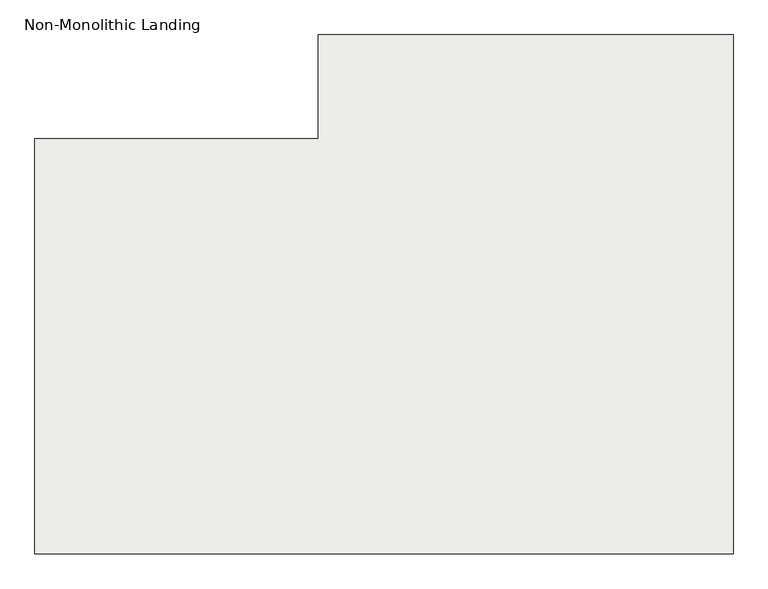
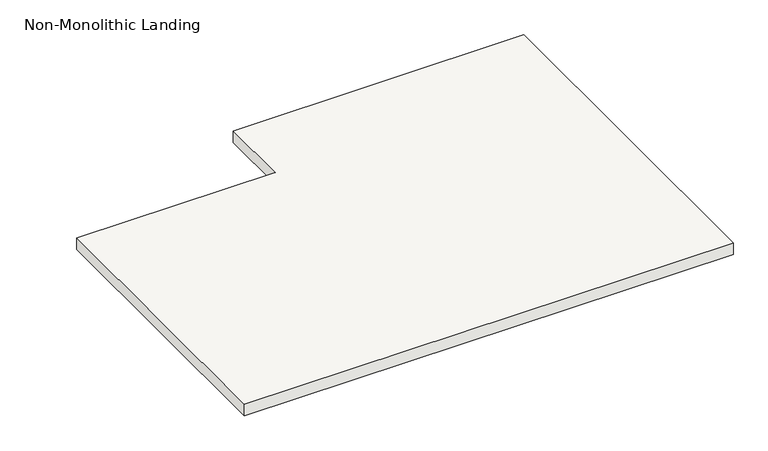
"""IFC4 building model written with IfcOpenShell, lengths in millimetres: slab geometry, Non-Monolithic Landing."""

import ifcopenshell
import ifcopenshell.guid

model = None  # the IFC model being written
_history = None  # IfcOwnerHistory: only IFC2X3 demands one
_inside = {}  # id of a spatial element -> (the spatial element, [elements in it])
_under = {}  # id of a project, library or spatial element -> (it, [spatial elements below it])
_declared = {}  # id of a project -> (the project, [libraries it declares])
_typed = {}  # id of a type object -> (the type object, [elements of that type])
_made_of = {}  # id of a material, layer set ... -> (it, [elements and type objects made of it])


def new_model(schema):
    """Start an empty IFC model of exactly this schema.

    Asked for "IFC4X3", IfcOpenShell would pick the latest addendum, in which some entities
    have other attributes; the version numbers below select the first issue.
    IFC2X3 requires an IfcOwnerHistory on every rooted entity: one is made here for all.
    """
    global model, _history
    if schema == "IFC4X3":
        model = ifcopenshell.file(schema_version=(4, 3, 0, 0))
    else:
        model = ifcopenshell.file(schema=schema)
    _inside.clear()
    _under.clear()
    _declared.clear()
    _typed.clear()
    _made_of.clear()
    _history = None
    if model.schema == "IFC2X3":
        org = make("IfcOrganization", Name="unknown")
        user = make(
            "IfcPersonAndOrganization",
            ThePerson=make("IfcPerson", FamilyName="unknown"),
            TheOrganization=org,
        )
        app = make(
            "IfcApplication",
            ApplicationDeveloper=org,
            Version="unknown",
            ApplicationFullName="unknown",
            ApplicationIdentifier="unknown",
        )
        _history = make(
            "IfcOwnerHistory",
            OwningUser=user,
            OwningApplication=app,
            ChangeAction="ADDED",
            CreationDate=0,
        )
    return model


def make(cls, **values):
    """One entity of the class cls with the attributes given. An attribute that is None is left unset."""
    return model.create_entity(
        cls, **{name: value for name, value in values.items() if value is not None}
    )


def rooted(cls, **values):
    """An entity with a GlobalId (a new one), such as an element, a storey or a relation."""
    return make(cls, GlobalId=ifcopenshell.guid.new(), OwnerHistory=_history, **values)


def si_unit(unit_type, name, prefix=None):
    """IfcSIUnit, for example si_unit("LENGTHUNIT", "METRE", prefix="MILLI")."""
    return make("IfcSIUnit", UnitType=unit_type, Prefix=prefix, Name=name)


def assignment(units):
    """IfcUnitAssignment: the units of a project."""
    return None if units is None else make("IfcUnitAssignment", Units=units)


def point(xyz):
    """IfcCartesianPoint."""
    return None if xyz is None else make("IfcCartesianPoint", Coordinates=xyz)


def direction(xyz):
    """IfcDirection."""
    return None if xyz is None else make("IfcDirection", DirectionRatios=xyz)


def frame(location, z_axis=None, x_axis=None):
    """IfcAxis2Placement3D, a coordinate frame: its origin and axes. An axis left out is left unset."""
    return make(
        "IfcAxis2Placement3D",
        Location=point(location),
        Axis=direction(z_axis),
        RefDirection=direction(x_axis),
    )


def origin():
    """The frame at (0, 0, 0) with its axes left unset."""
    return frame((0.0, 0.0, 0.0))


def place(relative_to, where):
    """IfcLocalPlacement: puts the frame where relative to a parent placement (None: the world)."""
    return make(
        "IfcLocalPlacement", PlacementRelTo=relative_to, RelativePlacement=where
    )


def context(
    kind, dimensions, precision=None, world=None, true_north=None, identifier=None
):
    """IfcGeometricRepresentationContext, for example the 3D "Model" context."""
    return make(
        "IfcGeometricRepresentationContext",
        ContextIdentifier=identifier,
        ContextType=kind,
        CoordinateSpaceDimension=dimensions,
        Precision=precision,
        WorldCoordinateSystem=world,
        TrueNorth=true_north,
    )


def project(units=None, contexts=None):
    """IfcProject with its units and contexts."""
    return rooted(
        "IfcProject",
        Name="project",
        RepresentationContexts=contexts,
        UnitsInContext=assignment(units),
    )


def spatial(cls, under=None, at=None, **own):
    """A site, building, storey or space (cls), placed at a placement, below another one or the project."""
    s = rooted(cls, ObjectPlacement=at, **own)
    if under is not None:
        _under.setdefault(under.id(), (under, []))[1].append(s)
    return s


def polyline(points):
    """IfcPolyline through the points."""
    return make("IfcPolyline", Points=[point(p) for p in points])


def outline(outer, holes=None, kind="AREA"):
    """IfcArbitraryClosedProfileDef: a profile drawn as a closed curve; with holes, ...WithVoids."""
    if holes is None:
        return make("IfcArbitraryClosedProfileDef", ProfileType=kind, OuterCurve=outer)
    return make(
        "IfcArbitraryProfileDefWithVoids",
        ProfileType=kind,
        OuterCurve=outer,
        InnerCurves=holes,
    )


def extrude(swept, where, along, depth):
    """IfcExtrudedAreaSolid: the profile swept, set in the frame where, extruded along a direction by depth."""
    return make(
        "IfcExtrudedAreaSolid",
        SweptArea=swept,
        Position=where,
        ExtrudedDirection=direction(along),
        Depth=depth,
    )


def shape(context_of_items, identifier, shape_type, items):
    """IfcShapeRepresentation: the items that make up one representation, for example the "Body"."""
    return make(
        "IfcShapeRepresentation",
        ContextOfItems=context_of_items,
        RepresentationIdentifier=identifier,
        RepresentationType=shape_type,
        Items=items,
    )


def source(mapping_origin, context_of_items, identifier, shape_type, items):
    """IfcRepresentationMap: a shape defined once, which mapped items show again and again."""
    return make(
        "IfcRepresentationMap",
        MappingOrigin=mapping_origin,
        MappedRepresentation=shape(context_of_items, identifier, shape_type, items),
    )


def transform(
    local_origin,
    x_axis=None,
    y_axis=None,
    z_axis=None,
    scale=None,
    scale2=None,
    scale3=None,
    uniform=True,
):
    """IfcCartesianTransformationOperator3D, or its non-uniform kind. x_axis, y_axis, z_axis: its Axis1, 2, 3."""
    if uniform:
        return make(
            "IfcCartesianTransformationOperator3D",
            Axis1=direction(x_axis),
            Axis2=direction(y_axis),
            LocalOrigin=point(local_origin),
            Scale=scale,
            Axis3=direction(z_axis),
        )
    return make(
        "IfcCartesianTransformationOperator3DnonUniform",
        Axis1=direction(x_axis),
        Axis2=direction(y_axis),
        LocalOrigin=point(local_origin),
        Scale=scale,
        Axis3=direction(z_axis),
        Scale2=scale2,
        Scale3=scale3,
    )


def mapped(mapping_source, mapping_target):
    """IfcMappedItem: shows the shape of a source again, moved by a transform."""
    return make(
        "IfcMappedItem", MappingSource=mapping_source, MappingTarget=mapping_target
    )


def made_of(thing, what):
    """Note that an element or type object is made of a material, layer set ...; save() writes the relation."""
    if what is not None:
        _made_of.setdefault(what.id(), (what, []))[1].append(thing)
    return thing


def element(
    cls,
    number,
    at=None,
    inside=None,
    cuts=None,
    type_object=None,
    material=None,
    context=None,
    identifier="Body",
    shape_type=None,
    held_by="IfcProductDefinitionShape",
    body=None,
    shapes=None,
    **own,
):
    """One element of the class cls, such as IfcWall. Its Tag is "e" and its number.

    at: its placement. inside: the storey or other place that contains it. cuts: it is an
    opening in that element (IfcRelVoidsElement). A single representation is given by context,
    identifier, shape_type and body (its items); several are given by shapes. held_by: the class
    of the entity that holds the representations. save() writes the other relations.
    """
    e = rooted(cls, Tag="e%d" % number, ObjectPlacement=at, **own)
    if body is not None:
        shapes = [shape(context, identifier, shape_type, body)]
    if shapes is not None:
        e.Representation = make(held_by, Representations=shapes)
    if inside is not None:
        _inside.setdefault(inside.id(), (inside, []))[1].append(e)
    if cuts is not None:
        rooted(
            "IfcRelVoidsElement", RelatingBuildingElement=cuts, RelatedOpeningElement=e
        )
    if type_object is not None:
        _typed.setdefault(type_object.id(), (type_object, []))[1].append(e)
    return made_of(e, material)


def aggregate(whole, parts):
    """IfcRelAggregates: a whole, such as a stair, and the parts it consists of."""
    return rooted("IfcRelAggregates", RelatingObject=whole, RelatedObjects=parts)


def save(model, path):
    """Write the relations noted so far, then the file.

    IfcRelAggregates (storeys below a building ...), IfcRelContainedInSpatialStructure (elements
    in a storey), IfcRelDefinesByType, IfcRelAssociatesMaterial and IfcRelDeclares: one each for
    every whole, place, type object, material and project.
    """
    for whole, parts in _under.values():
        aggregate(whole, parts)
    for where, things in _inside.values():
        rooted(
            "IfcRelContainedInSpatialStructure",
            RelatedElements=things,
            RelatingStructure=where,
        )
    for kind, things in _typed.values():
        rooted("IfcRelDefinesByType", RelatedObjects=things, RelatingType=kind)
    for what, things in _made_of.values():
        rooted("IfcRelAssociatesMaterial", RelatedObjects=things, RelatingMaterial=what)
    for by, libraries in _declared.values():
        rooted("IfcRelDeclares", RelatingContext=by, RelatedDefinitions=libraries)
    model.write(path)


def non_monolithic_landing_fffc1bba(model_context):
    return source(origin(), model_context, "Body", "SweptSolid", [
        extrude(outline(polyline([(22758.5156953, -2193.8863261), (22758.5156953, -3693.8863261), (20739.4907974, -3693.8863261), (20739.4907974, -2493.8863261), (21558.5156953, -2493.8863261), (21558.5156953, -2193.8863261), (22758.5156953, -2193.8863261)])), frame((0.0, 0.0, 1450.0), z_axis=(0.0, 0.0, 1.0), x_axis=(1.0, 0.0, 0.0)), (0.0, 0.0, 1.0), 50.0),
    ])


if __name__ == "__main__":
    model = new_model("IFC4")
    model_context = context("Model", 3, world=origin())
    ifc_project = project(units=[si_unit("LENGTHUNIT", "METRE", prefix="MILLI")], contexts=[model_context])
    site = spatial("IfcSite", under=ifc_project)
    building = spatial("IfcBuilding", under=site)
    placement = place(None, origin())
    non_monolithic_landing_shape = non_monolithic_landing_fffc1bba(model_context)
    element("IfcSlab", 1, ObjectType="Non-Monolithic Landing", at=placement, inside=building, context=model_context, shape_type="MappedRepresentation", body=[
        mapped(non_monolithic_landing_shape, transform((0.0, 0.0, 0.0), x_axis=(1.0, 0.0, 0.0), y_axis=(0.0, 1.0, 0.0), z_axis=(0.0, 0.0, 1.0))),
    ])
    save(model, "model.ifc")
